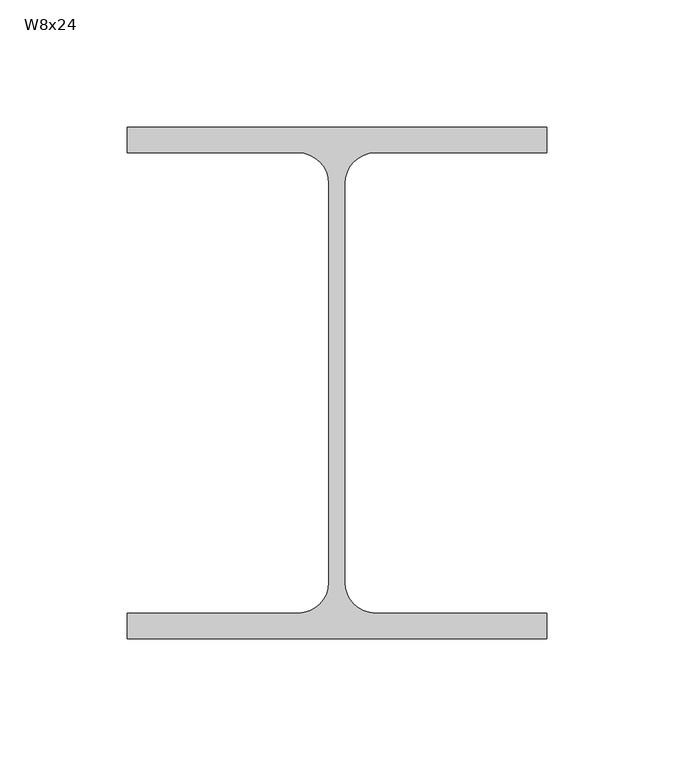
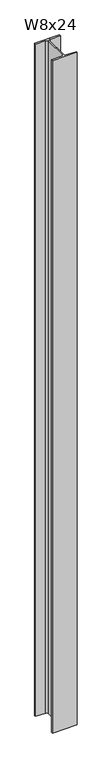
"""IFC4 building model written with IfcOpenShell, lengths in millimetres: column geometry, RME WF - Column : W8x24."""

from ifc_helpers import new_model, si_unit, point, frame, frame_2d, origin, place, context, project, spatial, polyline, circle_curve, trimmed, segment, composite_curve, outline, extrude, source, transform, mapped, element, save


def w8x24_f51a4e52(model_context):
    return source(origin(), model_context, "Body", "SweptSolid", [
        extrude(outline(composite_curve([segment(polyline([(82.55, 100.711), (82.55, 90.551), (15.1765, 90.551)]), True, "CONTINUOUS"), segment(trimmed(circle_curve(frame_2d((15.1765, 78.486)), 12.065), [point((15.1765, 90.551))], [point((3.1115, 78.486))], True, "CARTESIAN"), True, "CONTINUOUS"), segment(polyline([(3.1115, 78.486), (3.1115, -78.486)]), True, "CONTINUOUS"), segment(trimmed(circle_curve(frame_2d((15.1765, -78.486)), 12.065), [point((3.1115, -78.486))], [point((15.1765, -90.551))], True, "CARTESIAN"), True, "CONTINUOUS"), segment(polyline([(15.1765, -90.551), (82.55, -90.551), (82.55, -100.711), (-82.55, -100.711), (-82.55, -90.551), (-15.1765, -90.551)]), True, "CONTINUOUS"), segment(trimmed(circle_curve(frame_2d((-15.1765, -78.486)), 12.065), [point((-15.1765, -90.551))], [point((-3.1115, -78.486))], True, "CARTESIAN"), True, "CONTINUOUS"), segment(polyline([(-3.1115, -78.486), (-3.1115, 78.486)]), True, "CONTINUOUS"), segment(trimmed(circle_curve(frame_2d((-15.1765, 78.486)), 12.065), [point((-3.1115, 78.486))], [point((-15.1765, 90.551))], True, "CARTESIAN"), True, "CONTINUOUS"), segment(polyline([(-15.1765, 90.551), (-82.55, 90.551), (-82.55, 100.711), (82.55, 100.711)]), True, "CONTINUOUS")], self_intersect=False)), frame((0.0, 0.0, -203.2), z_axis=(0.0, 0.0, 1.0), x_axis=(1.0, 0.0, 0.0)), (0.0, 0.0, 1.0), 4699.0),
    ])


if __name__ == "__main__":
    model = new_model("IFC4")
    model_context = context("Model", 3, world=origin())
    ifc_project = project(units=[si_unit("LENGTHUNIT", "METRE", prefix="MILLI")], contexts=[model_context])
    site = spatial("IfcSite", under=ifc_project)
    building = spatial("IfcBuilding", under=site)
    placement = place(None, origin())
    w8x24_shape = w8x24_f51a4e52(model_context)
    element("IfcColumn", 1, ObjectType="RME WF - Column : W8x24", at=placement, inside=building, context=model_context, shape_type="MappedRepresentation", body=[
        mapped(w8x24_shape, transform((0.0, 0.0, 0.0), x_axis=(1.0, 0.0, 0.0), y_axis=(0.0, 1.0, 0.0), z_axis=(0.0, 0.0, 1.0))),
    ])
    save(model, "model.ifc")

# Revit data of these elements
# Type "RME WF - Column : W8x24"
#   Type Mark = "C1"
#   REINF TYPE [instance default] = ""
#   Nominal Size = "W16"
#   COL REMARKS [instance default] = ""
#   BP [instance default] = ""
#   Assembly Code = "B10"
#   W = 24
#   bf = 0' - 6 1/2"
#   d = 0' - 7.93"
#   k = 0' - 0 7/8"
#   kr = 0' - 0.475"
#   tf = 0' - 0.4"
#   tw = 0' - 0.245"
#   A = 0.0491667 SF
#   Structural Material [instance default] = Metal - Steel - ASTM A992
# Element 1 (IfcColumn, "RME WF - Column : W8x24")
#   Materials on its faces: "Metal - Steel - ASTM A992"
# Materials
#   "Metal - Steel - ASTM A992": class "Metal", colour RGB 255 128 0, transparency 0
